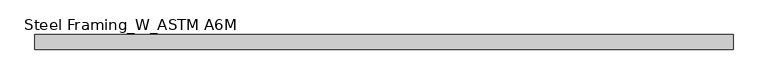
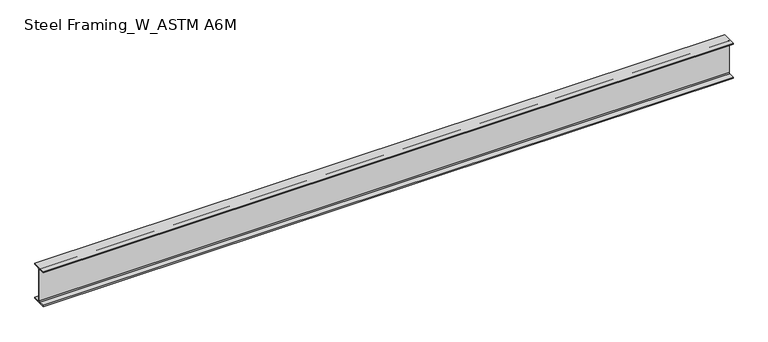
"""IFC4 building model written with IfcOpenShell, lengths in millimetres: beam geometry, Steel Framing_W_ASTM A6M : H_SB_AR_S02_W530x101_RB1."""

import ifcopenshell
import ifcopenshell.guid

model = None  # the IFC model being written
_history = None  # IfcOwnerHistory: only IFC2X3 demands one
_inside = {}  # id of a spatial element -> (the spatial element, [elements in it])
_under = {}  # id of a project, library or spatial element -> (it, [spatial elements below it])
_declared = {}  # id of a project -> (the project, [libraries it declares])
_typed = {}  # id of a type object -> (the type object, [elements of that type])
_made_of = {}  # id of a material, layer set ... -> (it, [elements and type objects made of it])


def new_model(schema):
    """Start an empty IFC model of exactly this schema.

    Asked for "IFC4X3", IfcOpenShell would pick the latest addendum, in which some entities
    have other attributes; the version numbers below select the first issue.
    IFC2X3 requires an IfcOwnerHistory on every rooted entity: one is made here for all.
    """
    global model, _history
    if schema == "IFC4X3":
        model = ifcopenshell.file(schema_version=(4, 3, 0, 0))
    else:
        model = ifcopenshell.file(schema=schema)
    _inside.clear()
    _under.clear()
    _declared.clear()
    _typed.clear()
    _made_of.clear()
    _history = None
    if model.schema == "IFC2X3":
        org = make("IfcOrganization", Name="unknown")
        user = make(
            "IfcPersonAndOrganization",
            ThePerson=make("IfcPerson", FamilyName="unknown"),
            TheOrganization=org,
        )
        app = make(
            "IfcApplication",
            ApplicationDeveloper=org,
            Version="unknown",
            ApplicationFullName="unknown",
            ApplicationIdentifier="unknown",
        )
        _history = make(
            "IfcOwnerHistory",
            OwningUser=user,
            OwningApplication=app,
            ChangeAction="ADDED",
            CreationDate=0,
        )
    return model


def make(cls, **values):
    """One entity of the class cls with the attributes given. An attribute that is None is left unset."""
    return model.create_entity(
        cls, **{name: value for name, value in values.items() if value is not None}
    )


def rooted(cls, **values):
    """An entity with a GlobalId (a new one), such as an element, a storey or a relation."""
    return make(cls, GlobalId=ifcopenshell.guid.new(), OwnerHistory=_history, **values)


def si_unit(unit_type, name, prefix=None):
    """IfcSIUnit, for example si_unit("LENGTHUNIT", "METRE", prefix="MILLI")."""
    return make("IfcSIUnit", UnitType=unit_type, Prefix=prefix, Name=name)


def assignment(units):
    """IfcUnitAssignment: the units of a project."""
    return None if units is None else make("IfcUnitAssignment", Units=units)


def point(xyz):
    """IfcCartesianPoint."""
    return None if xyz is None else make("IfcCartesianPoint", Coordinates=xyz)


def direction(xyz):
    """IfcDirection."""
    return None if xyz is None else make("IfcDirection", DirectionRatios=xyz)


def frame(location, z_axis=None, x_axis=None):
    """IfcAxis2Placement3D, a coordinate frame: its origin and axes. An axis left out is left unset."""
    return make(
        "IfcAxis2Placement3D",
        Location=point(location),
        Axis=direction(z_axis),
        RefDirection=direction(x_axis),
    )


def frame_2d(location, x_axis=None):
    """IfcAxis2Placement2D, a coordinate frame in the plane: its origin and x axis."""
    return make(
        "IfcAxis2Placement2D", Location=point(location), RefDirection=direction(x_axis)
    )


def origin():
    """The frame at (0, 0, 0) with its axes left unset."""
    return frame((0.0, 0.0, 0.0))


def place(relative_to, where):
    """IfcLocalPlacement: puts the frame where relative to a parent placement (None: the world)."""
    return make(
        "IfcLocalPlacement", PlacementRelTo=relative_to, RelativePlacement=where
    )


def context(
    kind, dimensions, precision=None, world=None, true_north=None, identifier=None
):
    """IfcGeometricRepresentationContext, for example the 3D "Model" context."""
    return make(
        "IfcGeometricRepresentationContext",
        ContextIdentifier=identifier,
        ContextType=kind,
        CoordinateSpaceDimension=dimensions,
        Precision=precision,
        WorldCoordinateSystem=world,
        TrueNorth=true_north,
    )


def project(units=None, contexts=None):
    """IfcProject with its units and contexts."""
    return rooted(
        "IfcProject",
        Name="project",
        RepresentationContexts=contexts,
        UnitsInContext=assignment(units),
    )


def spatial(cls, under=None, at=None, **own):
    """A site, building, storey or space (cls), placed at a placement, below another one or the project."""
    s = rooted(cls, ObjectPlacement=at, **own)
    if under is not None:
        _under.setdefault(under.id(), (under, []))[1].append(s)
    return s


def polyline(points):
    """IfcPolyline through the points."""
    return make("IfcPolyline", Points=[point(p) for p in points])


def circle_curve(where, radius):
    """IfcCircle in the frame where."""
    return make("IfcCircle", Position=where, Radius=radius)


def trimmed(basis, trim1, trim2, sense, master):
    """IfcTrimmedCurve: the piece of a basis curve between two trims."""
    return make(
        "IfcTrimmedCurve",
        BasisCurve=basis,
        Trim1=trim1,
        Trim2=trim2,
        SenseAgreement=sense,
        MasterRepresentation=master,
    )


def segment(curve, same_sense, transition):
    """IfcCompositeCurveSegment."""
    return make(
        "IfcCompositeCurveSegment",
        Transition=transition,
        SameSense=same_sense,
        ParentCurve=curve,
    )


def composite_curve(segments, self_intersect=None):
    """IfcCompositeCurve: segments joined end to end."""
    return make("IfcCompositeCurve", Segments=segments, SelfIntersect=self_intersect)


def outline(outer, holes=None, kind="AREA"):
    """IfcArbitraryClosedProfileDef: a profile drawn as a closed curve; with holes, ...WithVoids."""
    if holes is None:
        return make("IfcArbitraryClosedProfileDef", ProfileType=kind, OuterCurve=outer)
    return make(
        "IfcArbitraryProfileDefWithVoids",
        ProfileType=kind,
        OuterCurve=outer,
        InnerCurves=holes,
    )


def extrude(swept, where, along, depth):
    """IfcExtrudedAreaSolid: the profile swept, set in the frame where, extruded along a direction by depth."""
    return make(
        "IfcExtrudedAreaSolid",
        SweptArea=swept,
        Position=where,
        ExtrudedDirection=direction(along),
        Depth=depth,
    )


def shape(context_of_items, identifier, shape_type, items):
    """IfcShapeRepresentation: the items that make up one representation, for example the "Body"."""
    return make(
        "IfcShapeRepresentation",
        ContextOfItems=context_of_items,
        RepresentationIdentifier=identifier,
        RepresentationType=shape_type,
        Items=items,
    )


def source(mapping_origin, context_of_items, identifier, shape_type, items):
    """IfcRepresentationMap: a shape defined once, which mapped items show again and again."""
    return make(
        "IfcRepresentationMap",
        MappingOrigin=mapping_origin,
        MappedRepresentation=shape(context_of_items, identifier, shape_type, items),
    )


def transform(
    local_origin,
    x_axis=None,
    y_axis=None,
    z_axis=None,
    scale=None,
    scale2=None,
    scale3=None,
    uniform=True,
):
    """IfcCartesianTransformationOperator3D, or its non-uniform kind. x_axis, y_axis, z_axis: its Axis1, 2, 3."""
    if uniform:
        return make(
            "IfcCartesianTransformationOperator3D",
            Axis1=direction(x_axis),
            Axis2=direction(y_axis),
            LocalOrigin=point(local_origin),
            Scale=scale,
            Axis3=direction(z_axis),
        )
    return make(
        "IfcCartesianTransformationOperator3DnonUniform",
        Axis1=direction(x_axis),
        Axis2=direction(y_axis),
        LocalOrigin=point(local_origin),
        Scale=scale,
        Axis3=direction(z_axis),
        Scale2=scale2,
        Scale3=scale3,
    )


def mapped(mapping_source, mapping_target):
    """IfcMappedItem: shows the shape of a source again, moved by a transform."""
    return make(
        "IfcMappedItem", MappingSource=mapping_source, MappingTarget=mapping_target
    )


def made_of(thing, what):
    """Note that an element or type object is made of a material, layer set ...; save() writes the relation."""
    if what is not None:
        _made_of.setdefault(what.id(), (what, []))[1].append(thing)
    return thing


def element(
    cls,
    number,
    at=None,
    inside=None,
    cuts=None,
    type_object=None,
    material=None,
    context=None,
    identifier="Body",
    shape_type=None,
    held_by="IfcProductDefinitionShape",
    body=None,
    shapes=None,
    **own,
):
    """One element of the class cls, such as IfcWall. Its Tag is "e" and its number.

    at: its placement. inside: the storey or other place that contains it. cuts: it is an
    opening in that element (IfcRelVoidsElement). A single representation is given by context,
    identifier, shape_type and body (its items); several are given by shapes. held_by: the class
    of the entity that holds the representations. save() writes the other relations.
    """
    e = rooted(cls, Tag="e%d" % number, ObjectPlacement=at, **own)
    if body is not None:
        shapes = [shape(context, identifier, shape_type, body)]
    if shapes is not None:
        e.Representation = make(held_by, Representations=shapes)
    if inside is not None:
        _inside.setdefault(inside.id(), (inside, []))[1].append(e)
    if cuts is not None:
        rooted(
            "IfcRelVoidsElement", RelatingBuildingElement=cuts, RelatedOpeningElement=e
        )
    if type_object is not None:
        _typed.setdefault(type_object.id(), (type_object, []))[1].append(e)
    return made_of(e, material)


def aggregate(whole, parts):
    """IfcRelAggregates: a whole, such as a stair, and the parts it consists of."""
    return rooted("IfcRelAggregates", RelatingObject=whole, RelatedObjects=parts)


def save(model, path):
    """Write the relations noted so far, then the file.

    IfcRelAggregates (storeys below a building ...), IfcRelContainedInSpatialStructure (elements
    in a storey), IfcRelDefinesByType, IfcRelAssociatesMaterial and IfcRelDeclares: one each for
    every whole, place, type object, material and project.
    """
    for whole, parts in _under.values():
        aggregate(whole, parts)
    for where, things in _inside.values():
        rooted(
            "IfcRelContainedInSpatialStructure",
            RelatedElements=things,
            RelatingStructure=where,
        )
    for kind, things in _typed.values():
        rooted("IfcRelDefinesByType", RelatedObjects=things, RelatingType=kind)
    for what, things in _made_of.values():
        rooted("IfcRelAssociatesMaterial", RelatedObjects=things, RelatingMaterial=what)
    for by, libraries in _declared.values():
        rooted("IfcRelDeclares", RelatingContext=by, RelatedDefinitions=libraries)
    model.write(path)


def steel_framing_w_astm_a6m_a5cbddeb(model_context):
    return source(origin(), model_context, "Body", "SweptSolid", [
        extrude(outline(composite_curve([segment(polyline([(105.0, -250.6), (105.0, -268.0), (-105.0, -268.0), (-105.0, -250.6), (-18.25, -250.6)]), True, "CONTINUOUS"), segment(trimmed(circle_curve(frame_2d((-18.25, -237.8)), 12.8), [point((-18.25, -250.6))], [point((-5.45, -237.8))], True, "CARTESIAN"), True, "CONTINUOUS"), segment(polyline([(-5.45, -237.8), (-5.45, 237.8)]), True, "CONTINUOUS"), segment(trimmed(circle_curve(frame_2d((-18.25, 237.8)), 12.8), [point((-5.45, 237.8))], [point((-18.25, 250.6))], True, "CARTESIAN"), True, "CONTINUOUS"), segment(polyline([(-18.25, 250.6), (-105.0, 250.6), (-105.0, 268.0), (105.0, 268.0), (105.0, 250.6), (18.25, 250.6)]), True, "CONTINUOUS"), segment(trimmed(circle_curve(frame_2d((18.25, 237.8)), 12.8), [point((18.25, 250.6))], [point((5.45, 237.8))], True, "CARTESIAN"), True, "CONTINUOUS"), segment(polyline([(5.45, 237.8), (5.45, -237.8)]), True, "CONTINUOUS"), segment(trimmed(circle_curve(frame_2d((18.25, -237.8)), 12.8), [point((5.45, -237.8))], [point((18.25, -250.6))], True, "CARTESIAN"), True, "CONTINUOUS"), segment(polyline([(18.25, -250.6), (105.0, -250.6)]), True, "CONTINUOUS")], self_intersect=False)), frame((-5000.0, 0.0, 0.0), z_axis=(1.0, 0.0, 0.0), x_axis=(0.0, 1.0, 0.0)), (0.0, 0.0, 1.0), 10000.0),
    ])


if __name__ == "__main__":
    model = new_model("IFC4")
    model_context = context("Model", 3, world=origin())
    ifc_project = project(units=[si_unit("LENGTHUNIT", "METRE", prefix="MILLI")], contexts=[model_context])
    site = spatial("IfcSite", under=ifc_project)
    building = spatial("IfcBuilding", under=site)
    placement = place(None, origin())
    steel_framing_w_astm_a6m_shape = steel_framing_w_astm_a6m_a5cbddeb(model_context)
    element("IfcBeam", 1, ObjectType="Steel Framing_W_ASTM A6M : H_SB_AR_S02_W530x101_RB1", at=placement, inside=building, context=model_context, shape_type="MappedRepresentation", body=[
        mapped(steel_framing_w_astm_a6m_shape, transform((0.0, 0.0, 0.0), x_axis=(1.0, 0.0, 0.0), y_axis=(0.0, 1.0, 0.0), z_axis=(0.0, 0.0, 1.0))),
    ])
    save(model, "model.ifc")

# Revit data of these elements
# Type "Steel Framing_W_ASTM A6M : H_SB_AR_S02_W530x101_RB1"
#   Section Name Key = "W21x68"
#   Width = 21.0 cm
#   Web Thickness = 1.09 cm
#   Web Fillet = 1.28 cm
#   Warping Constant = 1820000.0 cm⁶
#   Torsional Moment of Inertia = 102.00 cm⁴
#   Section Area = 129.0 cm²
#   Plastic Modulus weak axis = 400.0 cm³
#   Plastic Modulus strong axis = 2620.0 cm³
#   Perimeter = 1.87 m²/m
#   Nominal Weight = 101.00 kgf/m
#   Moment of Inertia weak axis = 2690.00 cm⁴
#   Moment of Inertia strong axis = 61600.00 cm⁴
#   Height = 53.6 cm
#   Flange Thickness = 1.74 cm
#   Elastic Modulus weak axis = 257.0 cm³
#   Elastic Modulus strong axis = 2290.0 cm³
#   Centroid Vertical = 26.8 cm
#   Centroid Horizontal = 10.5 cm
#   Length [instance default] = 1500 mm
#   Structural Material [instance default] = Steel, 45-345
#   Bolt Spacing = 0
#   Assembly Code = ""
# Element 1 (IfcBeam, "Steel Framing_W_ASTM A6M : H_SB_AR_S02_W530x101_RB1")
#   Materials on its faces: "Steel, 45-345"
# Materials
#   "Steel, 45-345": class "Metal", colour RGB 189 187 185, transparency 0, Description = "Steel 345 MPa", Cost = 0
